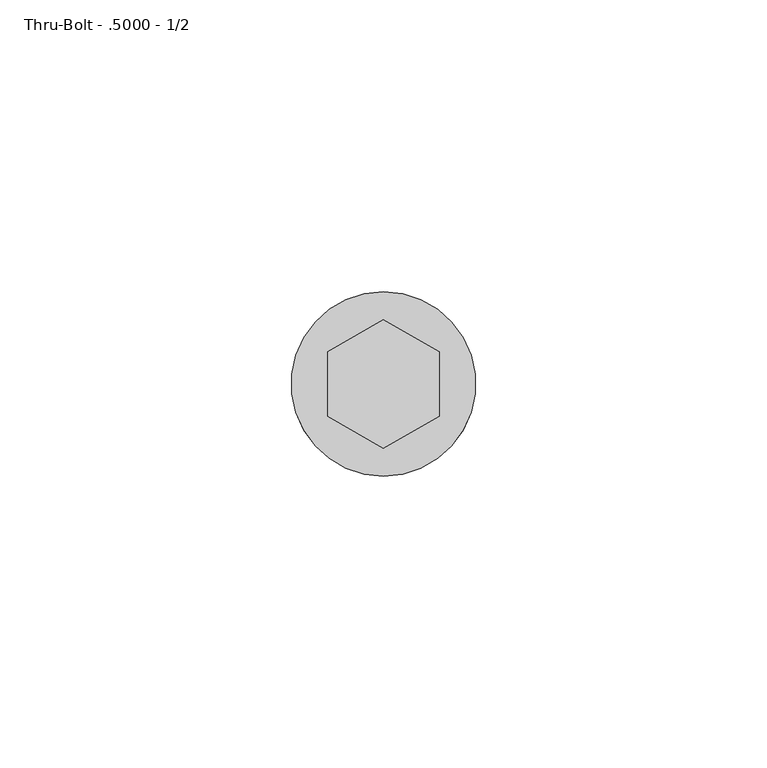
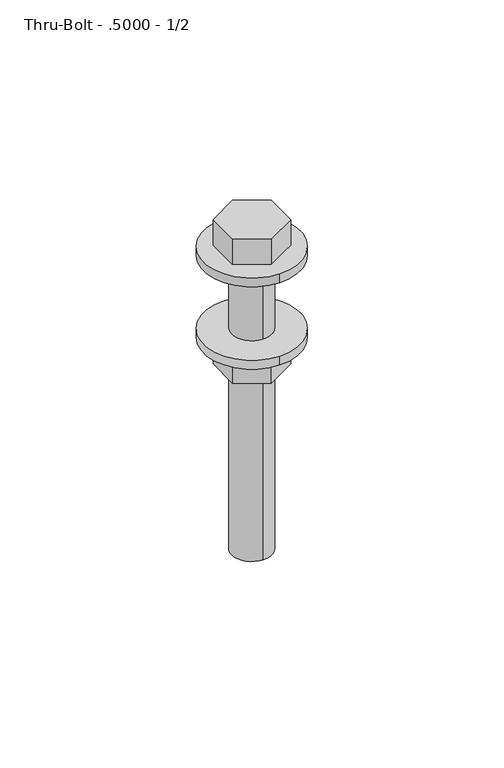
"""IFC4 building model written with IfcOpenShell, lengths in millimetres: fastener geometry, 060523 - W_P_C - Fastenings - Generic : Thru-Bolt - .5000 - 1/2."""

from ifc_helpers import new_model, si_unit, point, frame, origin, origin_with_axes, origin_2d, place, context, project, spatial, polyline, circle_curve, trimmed, segment, composite_curve, outline, extrude, source, transform, mapped, element, save


def thru_bolt_5000_1_2_3a1a67ea(model_context):
    return source(origin(), model_context, "Body", "SweptSolid", [
        extrude(outline(composite_curve([segment(trimmed(circle_curve(origin_2d(), 15.7757813), [point((0.0, 15.7757812))], [point((0.0, -15.7757813))], False, "CARTESIAN"), True, "CONTINUOUS"), segment(trimmed(circle_curve(origin_2d(), 15.7757813), [point((0.0, -15.7757813))], [point((0.0, 15.7757812))], False, "CARTESIAN"), True, "CONTINUOUS")], self_intersect=False)), origin_with_axes(), (0.0, 0.0, 1.0), 3.0757812),
        extrude(outline(composite_curve([segment(trimmed(circle_curve(origin_2d(), 15.7757813), [point((0.0, 15.7757812))], [point((0.0, -15.7757813))], False, "CARTESIAN"), True, "CONTINUOUS"), segment(trimmed(circle_curve(origin_2d(), 15.7757813), [point((0.0, -15.7757813))], [point((0.0, 15.7757812))], False, "CARTESIAN"), True, "CONTINUOUS")], self_intersect=False)), frame((0.0, 0.0, -28.4757813), z_axis=(0.0, 0.0, 1.0), x_axis=(1.0, 0.0, 0.0)), (0.0, 0.0, 1.0), 3.0757812),
        extrude(outline(polyline([(-9.525, -5.4992613), (-9.525, 5.4992613), (0.0, 10.9985226), (9.525, 5.4992613), (9.525, -5.4992613), (0.0, -10.9985226), (-9.525, -5.4992613)])), frame((0.0, 0.0, -37.703125), z_axis=(0.0, 0.0, 1.0), x_axis=(1.0, 0.0, 0.0)), (0.0, 0.0, 1.0), 9.2273437),
        extrude(outline(polyline([(-9.525, 5.4992613), (0.0, 10.9985226), (9.525, 5.4992613), (9.525, -5.4992613), (0.0, -10.9985226), (-9.525, -5.4992613), (-9.525, 5.4992613)])), frame((0.0, 0.0, 3.0757813), z_axis=(0.0, 0.0, 1.0), x_axis=(1.0, 0.0, 0.0)), (0.0, 0.0, 1.0), 9.2273437),
        extrude(outline(composite_curve([segment(trimmed(circle_curve(origin_2d(), 6.5484375), [point((0.0, -6.5484375))], [point((0.0, 6.5484375))], False, "CARTESIAN"), True, "CONTINUOUS"), segment(trimmed(circle_curve(origin_2d(), 6.5484375), [point((0.0, 6.5484375))], [point((0.0, -6.5484375))], False, "CARTESIAN"), True, "CONTINUOUS")], self_intersect=False)), frame((0.0, 0.0, -101.6), z_axis=(0.0, 0.0, 1.0), x_axis=(1.0, 0.0, 0.0)), (0.0, 0.0, 1.0), 104.6757812),
    ])


if __name__ == "__main__":
    model = new_model("IFC4")
    model_context = context("Model", 3, world=origin())
    ifc_project = project(units=[si_unit("LENGTHUNIT", "METRE", prefix="MILLI")], contexts=[model_context])
    site = spatial("IfcSite", under=ifc_project)
    building = spatial("IfcBuilding", under=site)
    placement = place(None, origin())
    thru_bolt_5000_1_2_shape = thru_bolt_5000_1_2_3a1a67ea(model_context)
    element("IfcFastener", 1, ObjectType="060523 - W_P_C - Fastenings - Generic : Thru-Bolt - .5000 - 1/2", at=placement, inside=building, context=model_context, shape_type="MappedRepresentation", body=[
        mapped(thru_bolt_5000_1_2_shape, transform((0.0, 0.0, 0.0), x_axis=(1.0, 0.0, 0.0), y_axis=(0.0, 1.0, 0.0), z_axis=(0.0, 0.0, 1.0))),
    ])
    save(model, "model.ifc")

# Revit data of these elements
# Type "060523 - W_P_C - Fastenings - Generic : Thru-Bolt - .5000 - 1/2"
#   Washer_Thickness = 0' - 0 31/256"
#   Washer Radius = 0' - 0 159/256"
#   Washer Offset - Head = 0' - 0 31/256"
#   Washer Offset = 0' - 0 31/256"
#   Thickness_of_Substrate [instance default] = 0' - 1"
#   Side = 0' - 0 111/256"
#   Radius = 0' - 0 33/128"
#   Length [instance default] = 0' - 4"
#   Head Size = 0' - 0 3/4"
#   Head Radius = 0' - 0 3/8"
#   Head Height = 0' - 0 93/256"
#   Double Diameter = 0' - 1 1/32"
#   Diameter = 0' - 0 33/64"
#   Default Elevation = 4' - 0"
#   Washer_Nut_Visibility = yes
#   Washer_Head_Visibility = yes
#   Round_Head_Visibility = no
#   Point Visibility = no
#   Nut_Visibility = yes
#   Hex_Head_Visiblilty = yes
#   Washer Material = none
#   Bolt Material (Size) = AT SILL - FASTENER AT 24" O.C.
# Element 1 (IfcFastener, "060523 - W_P_C - Fastenings - Generic : Thru-Bolt - .5000 - 1/2")
#   Materials on its faces: "AT SILL - FASTENER AT 24\" O.C."
# Materials
#   "AT SILL - FASTENER AT 24\" O.C.": class "Generic", colour RGB 120 120 120, transparency 0, Cost = 0
